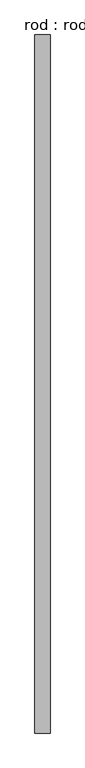
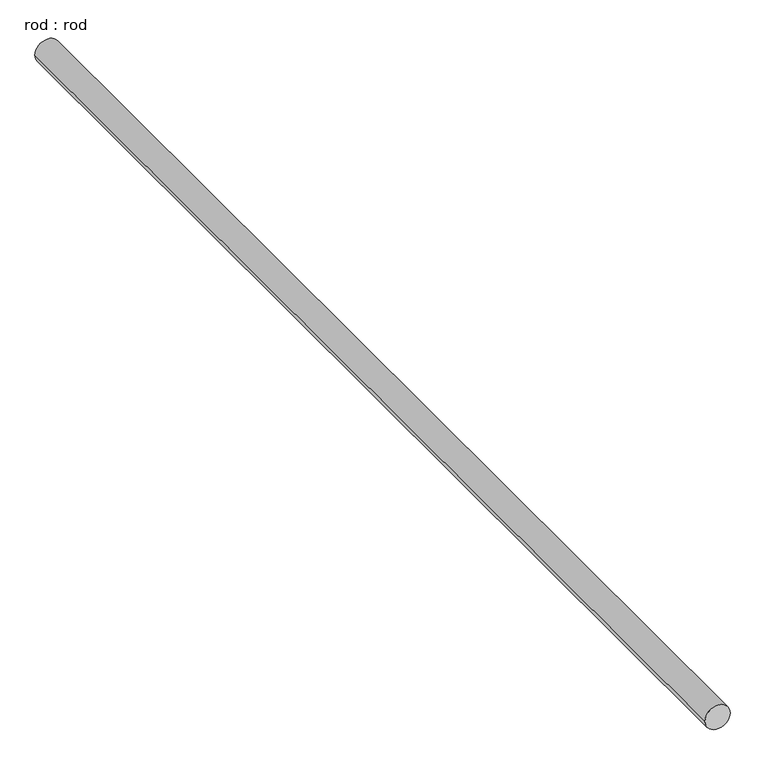
"""IFC4 building model written with IfcOpenShell, lengths in millimetres: proxy geometry, rod : rod."""

from ifc_helpers import new_model, si_unit, point, frame, frame_2d, origin, place, context, project, spatial, circle_curve, trimmed, segment, composite_curve, outline, extrude, source, transform, mapped, element, save


def rod_rod_9903d5c9(model_context):
    return source(origin(), model_context, "Body", "SweptSolid", [
        extrude(outline(composite_curve([segment(trimmed(circle_curve(frame_2d((0.0108462, 0.0)), 200.0), [point((0.0108462, 200.0))], [point((0.0108462, -200.0))], False, "CARTESIAN"), True, "CONTINUOUS"), segment(trimmed(circle_curve(frame_2d((0.0108462, 0.0)), 200.0), [point((0.0108462, -200.0))], [point((0.0108462, 200.0))], False, "CARTESIAN"), True, "CONTINUOUS")], self_intersect=False)), frame((0.0, -5149.7148564, 0.0), z_axis=(0.0, 1.0, 0.0), x_axis=(0.0, 0.0, 1.0)), (0.0, 0.0, 1.0), 18484.8869435),
    ])


if __name__ == "__main__":
    model = new_model("IFC4")
    model_context = context("Model", 3, world=origin())
    ifc_project = project(units=[si_unit("LENGTHUNIT", "METRE", prefix="MILLI")], contexts=[model_context])
    site = spatial("IfcSite", under=ifc_project)
    building = spatial("IfcBuilding", under=site)
    placement = place(None, origin())
    rod_rod_shape = rod_rod_9903d5c9(model_context)
    element("IfcBuildingElementProxy", 1, Name="rod : rod", ObjectType="rod : rod", at=placement, inside=building, context=model_context, shape_type="MappedRepresentation", body=[
        mapped(rod_rod_shape, transform((0.0, 0.0, 0.0), x_axis=(1.0, 0.0, 0.0), y_axis=(0.0, 1.0, 0.0), z_axis=(0.0, 0.0, 1.0))),
    ])
    save(model, "model.ifc")

# Revit data of these elements
# Type "rod : rod"
#   Default Elevation = 0
